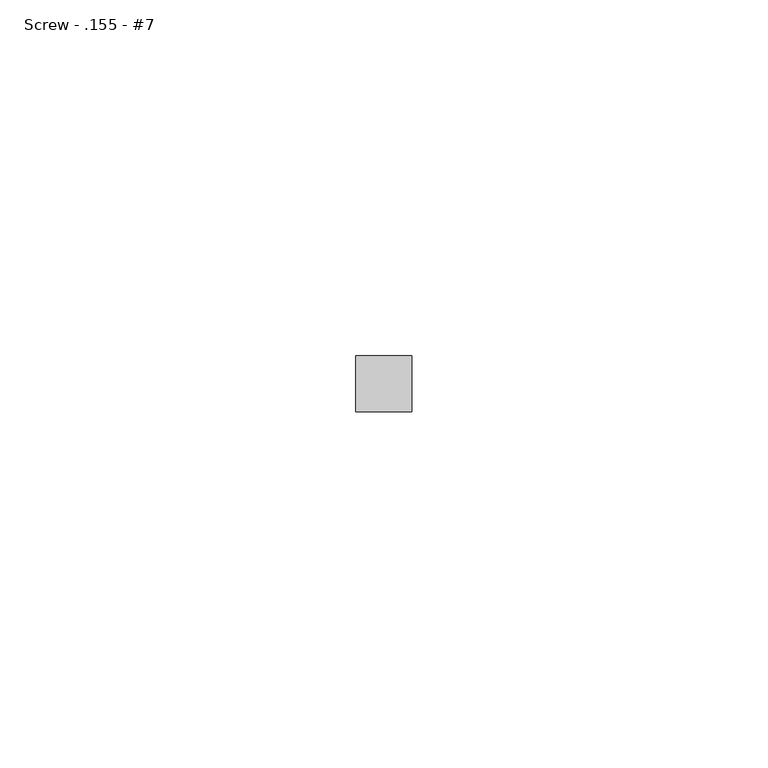
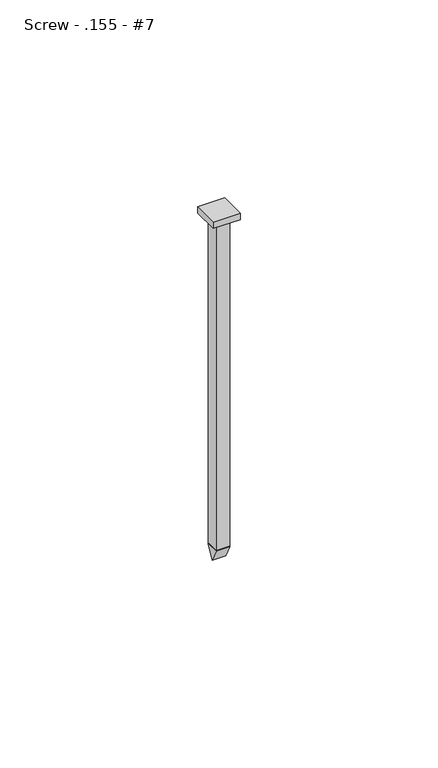
"""IFC4 building model written with IfcOpenShell, lengths in millimetres: fastener geometry, 060523 - W_P_C - Fastenings - Generic - SQUARE : Screw - .155 - #7."""

from ifc_helpers import new_model, si_unit, frame, origin, origin_with_axes, place, context, project, spatial, polyline, outline, extrude, source, transform, mapped, element, save


def screw_155_7_01879663(model_context):
    return source(origin(), model_context, "Body", "SweptSolid", [
        extrude(outline(polyline([(0.0, -105.537), (-1.9685, -101.6), (1.9685, -101.6), (0.0, -105.537)])), frame((-1.9685, 0.0, 0.0), z_axis=(1.0, 0.0, 0.0), x_axis=(0.0, 1.0, 0.0)), (0.0, 0.0, 1.0), 3.937),
        extrude(outline(polyline([(-3.937, -3.937), (-3.937, 3.937), (3.937, 3.937), (3.937, -3.937), (-3.937, -3.937)])), origin_with_axes(), (0.0, 0.0, 1.0), 1.9685),
        extrude(outline(polyline([(-1.9685, 1.9685), (1.9685, 1.9685), (1.9685, -1.9685), (-1.9685, -1.9685), (-1.9685, 1.9685)])), frame((0.0, 0.0, -101.6), z_axis=(0.0, 0.0, 1.0), x_axis=(1.0, 0.0, 0.0)), (0.0, 0.0, 1.0), 101.6),
    ])


if __name__ == "__main__":
    model = new_model("IFC4")
    model_context = context("Model", 3, world=origin())
    ifc_project = project(units=[si_unit("LENGTHUNIT", "METRE", prefix="MILLI")], contexts=[model_context])
    site = spatial("IfcSite", under=ifc_project)
    building = spatial("IfcBuilding", under=site)
    placement = place(None, origin())
    screw_155_7_shape = screw_155_7_01879663(model_context)
    element("IfcFastener", 1, ObjectType="060523 - W_P_C - Fastenings - Generic - SQUARE : Screw - .155 - #7", at=placement, inside=building, context=model_context, shape_type="MappedRepresentation", body=[
        mapped(screw_155_7_shape, transform((0.0, 0.0, 0.0), x_axis=(1.0, 0.0, 0.0), y_axis=(0.0, 1.0, 0.0), z_axis=(0.0, 0.0, 1.0))),
    ])
    save(model, "model.ifc")

# Revit data of these elements
# Type "060523 - W_P_C - Fastenings - Generic - SQUARE : Screw - .155 - #7"
#   Washer_Thickness = 0' - 0.00333"
#   Washer Radius = 0' - 0.0875"
#   Washer Offset - Head = 0' - 0"
#   Washer Offset = 0' - 0"
#   Thickness_of_Substrate [instance default] = 0' - 1"
#   Side = 0' - 0 37/64"
#   Radius = 0' - 0.0775"
#   Length [instance default] = 0' - 4"
#   Head Size = 0' - 1"
#   Head Radius = 0' - 0 1/2"
#   Head Height = 0' - 0.01"
#   Double Diameter = 0' - 0.31"
#   Diameter = 0' - 0.155"
#   Default Elevation = 4' - 0"
#   Washer_Nut_Visibility = no
#   Washer_Head_Visibility = no
#   Round_Head_Visibility = yes
#   Point Visibility = yes
#   Nut_Visibility = no
#   Hex_Head_Visiblilty = no
#   Washer Material = none
#   Bolt Material (Size) = AT SILL - FASTENER AT 24" O.C.
# Materials
#   "AT SILL - FASTENER AT 24\" O.C.": class "Generic", colour RGB 120 120 120, transparency 0, Cost = 0
